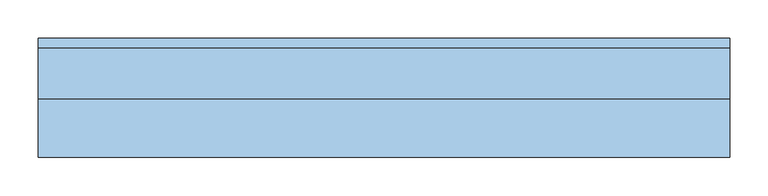
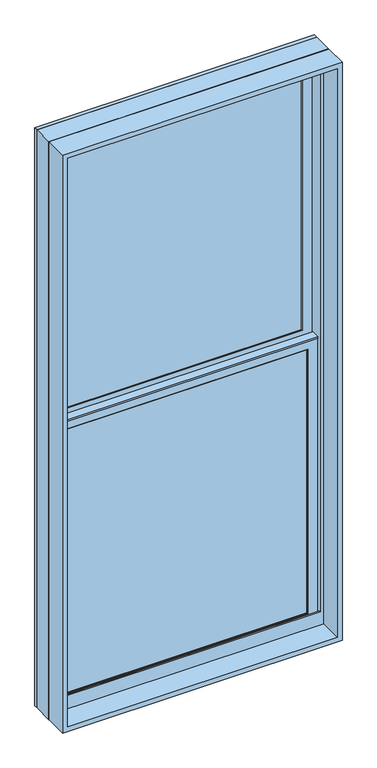
"""IFC4 building model written with IfcOpenShell, lengths in millimetres: window geometry, Window-Double_Hung-Marvin-Essential : ESDH3066."""

import ifcopenshell
import ifcopenshell.guid

model = None  # the IFC model being written
_history = None  # IfcOwnerHistory: only IFC2X3 demands one
_inside = {}  # id of a spatial element -> (the spatial element, [elements in it])
_under = {}  # id of a project, library or spatial element -> (it, [spatial elements below it])
_declared = {}  # id of a project -> (the project, [libraries it declares])
_typed = {}  # id of a type object -> (the type object, [elements of that type])
_made_of = {}  # id of a material, layer set ... -> (it, [elements and type objects made of it])


def new_model(schema):
    """Start an empty IFC model of exactly this schema.

    Asked for "IFC4X3", IfcOpenShell would pick the latest addendum, in which some entities
    have other attributes; the version numbers below select the first issue.
    IFC2X3 requires an IfcOwnerHistory on every rooted entity: one is made here for all.
    """
    global model, _history
    if schema == "IFC4X3":
        model = ifcopenshell.file(schema_version=(4, 3, 0, 0))
    else:
        model = ifcopenshell.file(schema=schema)
    _inside.clear()
    _under.clear()
    _declared.clear()
    _typed.clear()
    _made_of.clear()
    _history = None
    if model.schema == "IFC2X3":
        org = make("IfcOrganization", Name="unknown")
        user = make(
            "IfcPersonAndOrganization",
            ThePerson=make("IfcPerson", FamilyName="unknown"),
            TheOrganization=org,
        )
        app = make(
            "IfcApplication",
            ApplicationDeveloper=org,
            Version="unknown",
            ApplicationFullName="unknown",
            ApplicationIdentifier="unknown",
        )
        _history = make(
            "IfcOwnerHistory",
            OwningUser=user,
            OwningApplication=app,
            ChangeAction="ADDED",
            CreationDate=0,
        )
    return model


def make(cls, **values):
    """One entity of the class cls with the attributes given. An attribute that is None is left unset."""
    return model.create_entity(
        cls, **{name: value for name, value in values.items() if value is not None}
    )


def rooted(cls, **values):
    """An entity with a GlobalId (a new one), such as an element, a storey or a relation."""
    return make(cls, GlobalId=ifcopenshell.guid.new(), OwnerHistory=_history, **values)


def si_unit(unit_type, name, prefix=None):
    """IfcSIUnit, for example si_unit("LENGTHUNIT", "METRE", prefix="MILLI")."""
    return make("IfcSIUnit", UnitType=unit_type, Prefix=prefix, Name=name)


def assignment(units):
    """IfcUnitAssignment: the units of a project."""
    return None if units is None else make("IfcUnitAssignment", Units=units)


def point(xyz):
    """IfcCartesianPoint."""
    return None if xyz is None else make("IfcCartesianPoint", Coordinates=xyz)


def direction(xyz):
    """IfcDirection."""
    return None if xyz is None else make("IfcDirection", DirectionRatios=xyz)


def frame(location, z_axis=None, x_axis=None):
    """IfcAxis2Placement3D, a coordinate frame: its origin and axes. An axis left out is left unset."""
    return make(
        "IfcAxis2Placement3D",
        Location=point(location),
        Axis=direction(z_axis),
        RefDirection=direction(x_axis),
    )


def origin():
    """The frame at (0, 0, 0) with its axes left unset."""
    return frame((0.0, 0.0, 0.0))


def place(relative_to, where):
    """IfcLocalPlacement: puts the frame where relative to a parent placement (None: the world)."""
    return make(
        "IfcLocalPlacement", PlacementRelTo=relative_to, RelativePlacement=where
    )


def context(
    kind, dimensions, precision=None, world=None, true_north=None, identifier=None
):
    """IfcGeometricRepresentationContext, for example the 3D "Model" context."""
    return make(
        "IfcGeometricRepresentationContext",
        ContextIdentifier=identifier,
        ContextType=kind,
        CoordinateSpaceDimension=dimensions,
        Precision=precision,
        WorldCoordinateSystem=world,
        TrueNorth=true_north,
    )


def project(units=None, contexts=None):
    """IfcProject with its units and contexts."""
    return rooted(
        "IfcProject",
        Name="project",
        RepresentationContexts=contexts,
        UnitsInContext=assignment(units),
    )


def spatial(cls, under=None, at=None, **own):
    """A site, building, storey or space (cls), placed at a placement, below another one or the project."""
    s = rooted(cls, ObjectPlacement=at, **own)
    if under is not None:
        _under.setdefault(under.id(), (under, []))[1].append(s)
    return s


def polyline(points):
    """IfcPolyline through the points."""
    return make("IfcPolyline", Points=[point(p) for p in points])


def outline(outer, holes=None, kind="AREA"):
    """IfcArbitraryClosedProfileDef: a profile drawn as a closed curve; with holes, ...WithVoids."""
    if holes is None:
        return make("IfcArbitraryClosedProfileDef", ProfileType=kind, OuterCurve=outer)
    return make(
        "IfcArbitraryProfileDefWithVoids",
        ProfileType=kind,
        OuterCurve=outer,
        InnerCurves=holes,
    )


def extrude(swept, where, along, depth):
    """IfcExtrudedAreaSolid: the profile swept, set in the frame where, extruded along a direction by depth."""
    return make(
        "IfcExtrudedAreaSolid",
        SweptArea=swept,
        Position=where,
        ExtrudedDirection=direction(along),
        Depth=depth,
    )


def faces_of(points, faces, orient=None, outer=None):
    """IfcFace entities. A face is a list of loops; a loop is a list of indices into points, from 0.

    orient and outer hold one flag for each loop. By default every Orientation is true, the
    first loop of a face is its IfcFaceOuterBound and the others are IfcFaceBound.
    """
    made = []
    for i, loops in enumerate(faces):
        bounds = []
        for j, loop in enumerate(loops):
            is_outer = j == 0 if outer is None else outer[i][j]
            bounds.append(
                make(
                    "IfcFaceOuterBound" if is_outer else "IfcFaceBound",
                    Bound=make("IfcPolyLoop", Polygon=[points[k] for k in loop]),
                    Orientation=True if orient is None else orient[i][j],
                )
            )
        made.append(make("IfcFace", Bounds=bounds))
    return made


def faceted_brep(points, faces, orient=None, outer=None, voids=None):
    """IfcFacetedBrep: a solid bounded by flat faces; with voids (closed shells), ...WithVoids."""
    shared = [point(p) for p in points]
    hull = make("IfcClosedShell", CfsFaces=faces_of(shared, faces, orient, outer))
    if voids is None:
        return make("IfcFacetedBrep", Outer=hull)
    return make(
        "IfcFacetedBrepWithVoids",
        Outer=hull,
        Voids=[
            make(cls, CfsFaces=faces_of(shared, fs, o, b)) for cls, fs, o, b in voids
        ],
    )


def shape(context_of_items, identifier, shape_type, items):
    """IfcShapeRepresentation: the items that make up one representation, for example the "Body"."""
    return make(
        "IfcShapeRepresentation",
        ContextOfItems=context_of_items,
        RepresentationIdentifier=identifier,
        RepresentationType=shape_type,
        Items=items,
    )


def source(mapping_origin, context_of_items, identifier, shape_type, items):
    """IfcRepresentationMap: a shape defined once, which mapped items show again and again."""
    return make(
        "IfcRepresentationMap",
        MappingOrigin=mapping_origin,
        MappedRepresentation=shape(context_of_items, identifier, shape_type, items),
    )


def transform(
    local_origin,
    x_axis=None,
    y_axis=None,
    z_axis=None,
    scale=None,
    scale2=None,
    scale3=None,
    uniform=True,
):
    """IfcCartesianTransformationOperator3D, or its non-uniform kind. x_axis, y_axis, z_axis: its Axis1, 2, 3."""
    if uniform:
        return make(
            "IfcCartesianTransformationOperator3D",
            Axis1=direction(x_axis),
            Axis2=direction(y_axis),
            LocalOrigin=point(local_origin),
            Scale=scale,
            Axis3=direction(z_axis),
        )
    return make(
        "IfcCartesianTransformationOperator3DnonUniform",
        Axis1=direction(x_axis),
        Axis2=direction(y_axis),
        LocalOrigin=point(local_origin),
        Scale=scale,
        Axis3=direction(z_axis),
        Scale2=scale2,
        Scale3=scale3,
    )


def mapped(mapping_source, mapping_target):
    """IfcMappedItem: shows the shape of a source again, moved by a transform."""
    return make(
        "IfcMappedItem", MappingSource=mapping_source, MappingTarget=mapping_target
    )


def made_of(thing, what):
    """Note that an element or type object is made of a material, layer set ...; save() writes the relation."""
    if what is not None:
        _made_of.setdefault(what.id(), (what, []))[1].append(thing)
    return thing


def element(
    cls,
    number,
    at=None,
    inside=None,
    cuts=None,
    type_object=None,
    material=None,
    context=None,
    identifier="Body",
    shape_type=None,
    held_by="IfcProductDefinitionShape",
    body=None,
    shapes=None,
    **own,
):
    """One element of the class cls, such as IfcWall. Its Tag is "e" and its number.

    at: its placement. inside: the storey or other place that contains it. cuts: it is an
    opening in that element (IfcRelVoidsElement). A single representation is given by context,
    identifier, shape_type and body (its items); several are given by shapes. held_by: the class
    of the entity that holds the representations. save() writes the other relations.
    """
    e = rooted(cls, Tag="e%d" % number, ObjectPlacement=at, **own)
    if body is not None:
        shapes = [shape(context, identifier, shape_type, body)]
    if shapes is not None:
        e.Representation = make(held_by, Representations=shapes)
    if inside is not None:
        _inside.setdefault(inside.id(), (inside, []))[1].append(e)
    if cuts is not None:
        rooted(
            "IfcRelVoidsElement", RelatingBuildingElement=cuts, RelatedOpeningElement=e
        )
    if type_object is not None:
        _typed.setdefault(type_object.id(), (type_object, []))[1].append(e)
    return made_of(e, material)


def aggregate(whole, parts):
    """IfcRelAggregates: a whole, such as a stair, and the parts it consists of."""
    return rooted("IfcRelAggregates", RelatingObject=whole, RelatedObjects=parts)


def save(model, path):
    """Write the relations noted so far, then the file.

    IfcRelAggregates (storeys below a building ...), IfcRelContainedInSpatialStructure (elements
    in a storey), IfcRelDefinesByType, IfcRelAssociatesMaterial and IfcRelDeclares: one each for
    every whole, place, type object, material and project.
    """
    for whole, parts in _under.values():
        aggregate(whole, parts)
    for where, things in _inside.values():
        rooted(
            "IfcRelContainedInSpatialStructure",
            RelatedElements=things,
            RelatingStructure=where,
        )
    for kind, things in _typed.values():
        rooted("IfcRelDefinesByType", RelatedObjects=things, RelatingType=kind)
    for what, things in _made_of.values():
        rooted("IfcRelAssociatesMaterial", RelatedObjects=things, RelatingMaterial=what)
    for by, libraries in _declared.values():
        rooted("IfcRelDeclares", RelatingContext=by, RelatedDefinitions=libraries)
    model.write(path)


def window_3b7d5063(model_context):
    return source(origin(), model_context, "Body", "SolidModel", [
        extrude(outline(polyline([(140.7583333, 20.6375), (140.7583333, 15.875), (121.7083333, 15.875), (121.7083333, 20.6375), (140.7583333, 20.6375)])), frame((0.0, 0.0, 527.05), z_axis=(0.0, 0.0, 1.0), x_axis=(1.0, 0.0, 0.0)), (0.0, 0.0, 1.0), 908.05),
        extrude(outline(polyline([(-121.7083333, 20.6375), (-121.7083333, 15.875), (-140.7583333, 15.875), (-140.7583333, 20.6375), (-121.7083333, 20.6375)])), frame((0.0, 0.0, 527.05), z_axis=(0.0, 0.0, 1.0), x_axis=(1.0, 0.0, 0.0)), (0.0, 0.0, 1.0), 908.05),
        extrude(outline(polyline([(393.7, 20.6375), (393.7, 15.875), (-393.7, 15.875), (-393.7, 20.6375), (393.7, 20.6375)])), frame((0.0, 0.0, 971.55), z_axis=(0.0, 0.0, 1.0), x_axis=(1.0, 0.0, 0.0)), (0.0, 0.0, 1.0), 19.05),
        extrude(outline(polyline([(-140.7583333, 46.83125), (-140.7583333, 51.59375), (-121.7083333, 51.59375), (-121.7083333, 46.83125), (-140.7583333, 46.83125)])), frame((0.0, 0.0, 1473.2), z_axis=(0.0, 0.0, 1.0), x_axis=(1.0, 0.0, 0.0)), (0.0, 0.0, 1.0), 908.05),
        extrude(outline(polyline([(121.7083333, 46.83125), (121.7083333, 51.59375), (140.7583333, 51.59375), (140.7583333, 46.83125), (121.7083333, 46.83125)])), frame((0.0, 0.0, 1473.2), z_axis=(0.0, 0.0, 1.0), x_axis=(1.0, 0.0, 0.0)), (0.0, 0.0, 1.0), 908.05),
        extrude(outline(polyline([(-393.7, 46.83125), (-393.7, 51.59375), (393.7, 51.59375), (393.7, 46.83125), (-393.7, 46.83125)])), frame((0.0, 0.0, 1917.7), z_axis=(0.0, 0.0, 1.0), x_axis=(1.0, 0.0, 0.0)), (0.0, 0.0, 1.0), 19.05),
        extrude(outline(polyline([(140.7583333, 20.6375), (121.7083333, 20.6375), (121.7083333, 25.4), (140.7583333, 25.4), (140.7583333, 20.6375)])), frame((0.0, 0.0, 527.05), z_axis=(0.0, 0.0, 1.0), x_axis=(1.0, 0.0, 0.0)), (0.0, 0.0, 1.0), 908.05),
        extrude(outline(polyline([(-121.7083333, 20.6375), (-140.7583333, 20.6375), (-140.7583333, 25.4), (-121.7083333, 25.4), (-121.7083333, 20.6375)])), frame((0.0, 0.0, 527.05), z_axis=(0.0, 0.0, 1.0), x_axis=(1.0, 0.0, 0.0)), (0.0, 0.0, 1.0), 908.05),
        extrude(outline(polyline([(393.7, 20.6375), (-393.7, 20.6375), (-393.7, 25.4), (393.7, 25.4), (393.7, 20.6375)])), frame((0.0, 0.0, 971.55), z_axis=(0.0, 0.0, 1.0), x_axis=(1.0, 0.0, 0.0)), (0.0, 0.0, 1.0), 19.05),
        extrude(outline(polyline([(-140.7583333, 56.35625), (-121.7083333, 56.35625), (-121.7083333, 51.59375), (-140.7583333, 51.59375), (-140.7583333, 56.35625)])), frame((0.0, 0.0, 1473.2), z_axis=(0.0, 0.0, 1.0), x_axis=(1.0, 0.0, 0.0)), (0.0, 0.0, 1.0), 908.05),
        extrude(outline(polyline([(121.7083333, 56.35625), (140.7583333, 56.35625), (140.7583333, 51.59375), (121.7083333, 51.59375), (121.7083333, 56.35625)])), frame((0.0, 0.0, 1473.2), z_axis=(0.0, 0.0, 1.0), x_axis=(1.0, 0.0, 0.0)), (0.0, 0.0, 1.0), 908.05),
        extrude(outline(polyline([(-393.7, 56.35625), (393.7, 56.35625), (393.7, 51.59375), (-393.7, 51.59375), (-393.7, 56.35625)])), frame((0.0, 0.0, 1917.7), z_axis=(0.0, 0.0, 1.0), x_axis=(1.0, 0.0, 0.0)), (0.0, 0.0, 1.0), 19.05),
        faceted_brep([(-420.6875, 5.6780605, 1465.1351748), (-420.6875, 5.6780605, 1460.5), (420.6875, 5.6780605, 1460.5), (420.6875, 5.6780605, 1465.1351748), (-420.6875, 34.8118605, 1465.1351748), (420.6875, 34.8118605, 1465.1351748), (420.6875, 34.8118605, 1460.5), (-420.6875, 34.8118605, 1460.5), (-420.6875, 30.1625, 1460.5), (-420.6875, 30.1625, 500.0625), (-420.6875, 8.9241104, 500.0625), (-420.6875, 8.9241104, 1460.5), (420.6875, 8.9241104, 1460.5), (420.6875, 30.1625, 1460.5), (420.6875, 8.9241104, 500.0625), (420.6875, 30.1625, 500.0625), (-404.8034752, 11.90625, 1446.2034752), (-404.8034752, 30.1625, 1446.2034752), (404.8034752, 30.1625, 1446.2034752), (404.8034752, 11.90625, 1446.2034752), (-388.14375, 10.4662439, 1429.54375), (-388.14375, 11.90625, 1429.54375), (388.14375, 11.90625, 1429.54375), (388.14375, 10.4662439, 1429.54375), (389.6858834, 8.9241104, 1431.0858834), (-389.6858834, 8.9241104, 1431.0858834), (404.8034752, 30.1625, 515.9465248), (404.8034752, 11.90625, 515.9465248), (388.14375, 11.90625, 532.60625), (388.14375, 10.4662439, 532.60625), (389.6858834, 8.9241104, 531.0641166), (-404.8034752, 30.1625, 515.9465248), (-404.8034752, 11.90625, 515.9465248), (-388.14375, 11.90625, 532.60625), (-388.14375, 10.4662439, 532.60625), (-389.6858834, 8.9241104, 531.0641166)], [[[0, 1, 2, 3]], [[4, 5, 6, 7]], [[1, 0, 4, 7, 8, 9, 10, 11]], [[2, 1, 11, 12]], [[7, 6, 13, 8]], [[3, 2, 12, 14, 15, 13, 6, 5]], [[0, 3, 5, 4]], [[16, 17, 18, 19]], [[20, 21, 22, 23]], [[20, 23, 24, 25]], [[19, 18, 26, 27]], [[23, 22, 28, 29]], [[24, 23, 29, 30]], [[27, 26, 31, 32]], [[29, 28, 33, 34]], [[30, 29, 34, 35]], [[15, 14, 10, 9]], [[15, 9, 8, 13], [18, 17, 31, 26]], [[17, 16, 32, 31]], [[16, 19, 27, 32], [22, 21, 33, 28]], [[21, 20, 34, 33]], [[20, 25, 35, 34]], [[10, 14, 12, 11], [25, 24, 30, 35]]]),
        extrude(outline(polyline([(38.5955581, 1446.2125), (33.5778968, 1446.2125), (33.5778968, 1447.8), (39.9405976, 1447.8), (39.9405976, 1446.2125), (61.515625, 1446.2125), (47.6307501, 1442.8975159), (38.5955581, 1442.8975159), (38.5955581, 1446.2125)])), frame((-420.6875, 0.0, 0.0), z_axis=(1.0, 0.0, 0.0), x_axis=(0.0, 1.0, 0.0)), (0.0, 0.0, 1.0), 841.375),
        faceted_brep([(450.85, 0.0, 469.9), (450.85, 0.0, 2438.4), (-450.85, 0.0, 2438.4), (-450.85, 0.0, 469.9), (424.65625, 0.0, 531.01875), (-424.65625, 0.0, 531.01875), (-424.65625, 0.0, 2412.20625), (424.65625, 0.0, 2412.20625), (424.65625, 3.96875, 469.9), (-424.65625, 3.96875, 469.9), (-424.65625, 3.96875, 531.01875), (424.65625, 3.96875, 531.01875), (-450.85, 65.6828125, 469.9), (-424.65625, 65.6828125, 469.9), (424.65625, 65.6828125, 469.9), (450.85, 65.6828125, 469.9), (-450.85, 65.6828125, 2438.4), (450.85, 65.6828125, 2438.4), (424.65625, 65.6828125, 2412.20625), (-424.65625, 65.6828125, 2412.20625)], [[[0, 1, 2, 3], [4, 5, 6, 7]], [[8, 9, 10, 11]], [[5, 4, 11, 10]], [[0, 3, 12, 13, 9, 8, 14, 15]], [[13, 12, 16, 17, 15, 14, 18, 19]], [[13, 19, 6, 5, 10, 9]], [[7, 6, 19, 18]], [[18, 14, 8, 11, 4, 7]], [[1, 0, 15, 17]], [[2, 1, 17, 16]], [[3, 2, 16, 12]]]),
        faceted_brep([(424.65625, 30.1625, 1454.15), (423.06875, 30.1625, 1454.15), (423.06875, 30.1625, 494.2544613), (424.65625, 30.1625, 494.2544613), (-423.06875, 30.1625, 1454.15), (-424.65625, 30.1625, 1454.15), (-424.65625, 30.1625, 494.2544613), (-423.06875, 30.1625, 494.2544613), (423.06875, 63.5, 1454.15), (424.65625, 63.5, 1454.15), (424.65625, 63.5, 487.7743077), (423.06875, 63.5, 487.7743077), (-424.65625, 63.5, 1454.15), (-423.06875, 63.5, 1454.15), (-423.06875, 63.5, 487.7743077), (-424.65625, 63.5, 487.7743077), (435.9108932, 3.96875, 499.3460105), (435.9108932, 3.96875, 469.9), (435.9108932, 65.6828125, 469.9), (435.9108932, 65.6828125, 487.350012), (-435.9108932, 3.96875, 469.9), (-435.9108932, 3.96875, 499.3460105), (-435.9108932, 65.6828125, 487.350012), (-435.9108932, 65.6828125, 469.9), (435.9108932, 78.58125, 484.8428097), (-435.9108932, 78.58125, 484.8428097), (-433.8971252, 68.2348864, 486.8539391), (-415.93135, 68.2348864, 486.8539391), (-415.93135, 65.6828125, 487.350012), (415.93135, 65.6828125, 487.350012), (415.93135, 68.2348864, 486.8539391), (433.8971252, 68.2348864, 486.8539391), (-450.85, 65.6828125, 469.9), (-450.85, 78.5948249, 469.9), (450.85, 78.5948249, 469.9), (450.85, 65.6828125, 469.9), (-450.85, 78.58125, 2438.4), (450.85, 78.58125, 2438.4), (435.9108932, 78.58125, 2423.4608932), (-435.9108932, 78.58125, 2423.4608932), (-450.85, 65.6828125, 2438.4), (-433.8971252, 68.2348864, 2421.4471252), (433.8971252, 68.2348864, 2421.4471252), (415.93135, 68.2348864, 2403.48135), (-415.93135, 68.2348864, 2403.48135), (-415.93135, 65.6828125, 2403.48135), (415.93135, 65.6828125, 2403.48135), (450.85, 65.6828125, 2438.4)], [[[0, 1, 2, 3]], [[4, 5, 6, 7]], [[8, 9, 10, 11]], [[12, 13, 14, 15]], [[1, 8, 11, 2]], [[9, 0, 3, 10]], [[1, 0, 9, 8]], [[5, 4, 13, 12]], [[5, 12, 15, 6]], [[13, 4, 7, 14]], [[16, 17, 18, 19]], [[20, 21, 22, 23]], [[24, 25, 26, 27, 28, 22, 21, 16, 19, 29, 30, 31], [3, 2, 11, 10], [7, 6, 15, 14]], [[17, 16, 21, 20]], [[17, 20, 23, 32, 33, 34, 35, 18]], [[34, 33, 36, 37], [25, 24, 38, 39]], [[33, 32, 40, 36]], [[39, 41, 26, 25]], [[41, 42, 31, 30, 43, 44, 27, 26]], [[44, 45, 28, 27]], [[40, 32, 23, 22, 28, 45, 46, 29, 19, 18, 35, 47]], [[36, 40, 47, 37]], [[39, 38, 42, 41]], [[44, 43, 46, 45]], [[34, 37, 47, 35]], [[42, 38, 24, 31]], [[46, 43, 30, 29]]]),
        extrude(outline(polyline([(400.84375, 11.90625), (-400.84375, 11.90625), (-400.84375, 15.08125), (400.84375, 15.08125), (400.84375, 11.90625)])), frame((0.0, 0.0, 519.90625), z_axis=(0.0, 0.0, 1.0), x_axis=(1.0, 0.0, 0.0)), (0.0, 0.0, 1.0), 922.3375),
        extrude(outline(polyline([(400.84375, 42.8625), (-400.84375, 42.8625), (-400.84375, 46.0375), (400.84375, 46.0375), (400.84375, 42.8625)])), frame((0.0, 0.0, 1466.05625), z_axis=(0.0, 0.0, 1.0), x_axis=(1.0, 0.0, 0.0)), (0.0, 0.0, 1.0), 922.3375),
        faceted_brep([(-388.14375, 31.194477, 1429.54375), (-389.6858834, 32.7366104, 1431.0858834), (389.6858834, 32.7366104, 1431.0858834), (388.14375, 31.194477, 1429.54375), (-388.14375, 30.1625, 1429.54375), (388.14375, 30.1625, 1429.54375), (-420.6875, 32.7366104, 1462.0875), (-420.6875, 30.1625, 1462.0875), (420.6875, 30.1625, 1462.0875), (420.6875, 32.7366104, 1462.0875), (389.6858834, 32.7366104, 531.0641166), (388.14375, 31.194477, 532.60625), (388.14375, 30.1625, 532.60625), (420.6875, 30.1625, 500.0625), (420.6875, 32.7366104, 500.0625), (-389.6858834, 32.7366104, 531.0641166), (-388.14375, 31.194477, 532.60625), (-388.14375, 30.1625, 532.60625), (-420.6875, 30.1625, 500.0625), (-420.6875, 32.7366104, 500.0625)], [[[0, 1, 2, 3]], [[4, 0, 3, 5]], [[6, 7, 8, 9]], [[3, 2, 10, 11]], [[5, 3, 11, 12]], [[9, 8, 13, 14]], [[11, 10, 15, 16]], [[12, 11, 16, 17]], [[14, 13, 18, 19]], [[9, 14, 19, 6], [1, 15, 10, 2]], [[16, 15, 1, 0]], [[17, 16, 0, 4]], [[7, 18, 13, 8], [5, 12, 17, 4]], [[19, 18, 7, 6]]]),
        faceted_brep([(-404.8034752, 42.8625, 2392.3534752), (-404.8034752, 61.11875, 2392.3534752), (404.8034752, 61.11875, 2392.3534752), (404.8034752, 42.8625, 2392.3534752), (-388.14375, 41.4224939, 2375.69375), (-388.14375, 42.8625, 2375.69375), (388.14375, 42.8625, 2375.69375), (388.14375, 41.4224939, 2375.69375), (-389.6858834, 39.8803604, 2377.2358834), (389.6858834, 39.8803604, 2377.2358834), (-420.6875, 61.11875, 2408.2375), (-420.6875, 39.8803604, 2408.2375), (420.6875, 39.8803604, 2408.2375), (420.6875, 61.11875, 2408.2375), (404.8034752, 61.11875, 1462.0965248), (404.8034752, 42.8625, 1462.0965248), (388.14375, 42.8625, 1478.75625), (388.14375, 41.4224939, 1478.75625), (389.6858834, 39.8803604, 1477.2141166), (420.6875, 39.8803604, 1446.2125), (420.6875, 61.11875, 1446.2125), (-404.8034752, 61.11875, 1462.0965248), (-404.8034752, 42.8625, 1462.0965248), (-388.14375, 42.8625, 1478.75625), (-388.14375, 41.4224939, 1478.75625), (-389.6858834, 39.8803604, 1477.2141166), (-420.6875, 39.8803604, 1446.2125), (-420.6875, 61.11875, 1446.2125)], [[[0, 1, 2, 3]], [[4, 5, 6, 7]], [[8, 4, 7, 9]], [[10, 11, 12, 13]], [[3, 2, 14, 15]], [[7, 6, 16, 17]], [[9, 7, 17, 18]], [[13, 12, 19, 20]], [[15, 14, 21, 22]], [[17, 16, 23, 24]], [[18, 17, 24, 25]], [[20, 19, 26, 27]], [[13, 20, 27, 10], [1, 21, 14, 2]], [[22, 21, 1, 0]], [[3, 15, 22, 0], [5, 23, 16, 6]], [[24, 23, 5, 4]], [[25, 24, 4, 8]], [[11, 26, 19, 12], [9, 18, 25, 8]], [[27, 26, 11, 10]]]),
        faceted_brep([(-420.6875, 61.11875, 1446.2125), (-420.6875, 63.6928604, 1446.2125), (420.6875, 63.6928604, 1446.2125), (420.6875, 61.11875, 1446.2125), (-388.14375, 62.150727, 1478.75625), (-388.14375, 61.11875, 1478.75625), (388.14375, 61.11875, 1478.75625), (388.14375, 62.150727, 1478.75625), (-389.6858834, 63.6928604, 1477.2141166), (389.6858834, 63.6928604, 1477.2141166), (420.6875, 63.6928604, 2408.2375), (420.6875, 61.11875, 2408.2375), (388.14375, 61.11875, 2375.69375), (388.14375, 62.150727, 2375.69375), (389.6858834, 63.6928604, 2377.2358834), (-420.6875, 63.6928604, 2408.2375), (-420.6875, 61.11875, 2408.2375), (-388.14375, 61.11875, 2375.69375), (-388.14375, 62.150727, 2375.69375), (-389.6858834, 63.6928604, 2377.2358834)], [[[0, 1, 2, 3]], [[4, 5, 6, 7]], [[8, 4, 7, 9]], [[3, 2, 10, 11]], [[7, 6, 12, 13]], [[9, 7, 13, 14]], [[11, 10, 15, 16]], [[13, 12, 17, 18]], [[14, 13, 18, 19]], [[16, 15, 1, 0]], [[3, 11, 16, 0], [5, 17, 12, 6]], [[18, 17, 5, 4]], [[19, 18, 4, 8]], [[1, 15, 10, 2], [9, 14, 19, 8]]]),
        extrude(outline(polyline([(400.84375, 26.19375), (-400.84375, 26.19375), (-400.84375, 30.1625), (400.84375, 30.1625), (400.84375, 26.19375)])), frame((0.0, 0.0, 519.90625), z_axis=(0.0, 0.0, 1.0), x_axis=(1.0, 0.0, 0.0)), (0.0, 0.0, 1.0), 922.3375),
        extrude(outline(polyline([(400.84375, 57.15), (-400.84375, 57.15), (-400.84375, 61.11875), (400.84375, 61.11875), (400.84375, 57.15)])), frame((0.0, 0.0, 1466.05625), z_axis=(0.0, 0.0, 1.0), x_axis=(1.0, 0.0, 0.0)), (0.0, 0.0, 1.0), 922.3375),
        extrude(outline(polyline([(2438.4, 450.85), (2438.4, -450.85), (469.9, -450.85), (469.9, 450.85), (2438.4, 450.85)]), holes=[polyline([(2422.525, 434.975), (485.775, 434.975), (485.775, -434.975), (2422.525, -434.975), (2422.525, 434.975)])]), frame((0.0, -76.2, 0.0), z_axis=(0.0, 1.0, 0.0), x_axis=(0.0, 0.0, 1.0)), (0.0, 0.0, 1.0), 75.40625),
    ])


if __name__ == "__main__":
    model = new_model("IFC4")
    model_context = context("Model", 3, world=origin())
    ifc_project = project(units=[si_unit("LENGTHUNIT", "METRE", prefix="MILLI")], contexts=[model_context])
    site = spatial("IfcSite", under=ifc_project)
    building = spatial("IfcBuilding", under=site)
    placement = place(None, origin())
    window_shape = window_3b7d5063(model_context)
    element("IfcWindow", 1, ObjectType="Window-Double_Hung-Marvin-Essential : ESDH3066", at=placement, inside=building, context=model_context, shape_type="MappedRepresentation", body=[
        mapped(window_shape, transform((0.0, 0.0, 0.0), x_axis=(1.0, 0.0, 0.0), y_axis=(0.0, 1.0, 0.0), z_axis=(0.0, 0.0, 1.0))),
    ])
    save(model, "model.ifc")

# Revit data of these elements
# Type "Window-Double_Hung-Marvin-Essential : ESDH3066"
#   Type Mark = "86"
#   Window Type = "Essential Double Hung"
#   Product data url = "https://bimobject.com/marvin-windows-and-doors/product/marvin-dhwau"
#   Product Guid = "c4a96547-874c-4385-91dc-a058adc19d98"
#   Frame = "All Ultrex"
#   Egress Window = "Yes"
#   URL = "www.marvin.com"
#   Model = "ESDH3066"
#   Manufacturer = "Marvin Windows and Doors"
#   Label Egress = "EGRESS WDW"
#   Glass Type = "IG Low E II with Argon"
#   Design Pressure = "DP40"
#   Description = "3678 DBHG"
#   Analytic Construction = "<None>"
#   Prairie Corner Width = 0' - 4"
#   Prairie Corner Height = 0' - 4"
#   Egress Width = 2' - 8 9/16"
#   Egress Height = 2' - 10 27/128"
#   Rough Width = 3' - 0"
#   Rough Height = 6' - 6"
#   Nominal Width = 3' - 0"
#   Nominal Height = 6' - 6"
#   Inset to Installation Flange [instance default] = 0' - 1"
#   Height = 6' - 5 1/2"
#   Egress Area = 7.73607 SF
#   Default Head Height = 8' - 0"
#   Width = 2' - 11 1/2"
#   Daylight Area = 14.9894 SF
#   DLO Width = 2' - 6 9/16"
#   DLO Height = 2' - 11 5/16"
#   Muntins Top Sash = yes
#   Lites Wide Top Sash = 3
#   Lites Wide Bottom Sash = 3
#   Lites High Top Sash = 2
#   Lites High Bottom Sash = 2
#   Lite Cut Prairie 9 = no
#   Lite Cut HV Grid = yes
#   Muntins Bottom Sash = yes
#   Label Visibility = no
#   Jamb Extension Visibility = yes
#   Edition number = 1
#   Interior Material = Ultrex-Marvin-Stonewhite
#   Glazing Material = Glass-Marvin-IG Low E II with Argon
#   Cladding Material = Ultrex-Marvin-Pebblegray
#   Wall Closure = (empty or 0)
#   Assembly Code = ""
# Element 1 (IfcWindow, "Window-Double_Hung-Marvin-Essential : ESDH3066")
#   Materials on its faces: "Ultrex-Marvin-Pebblegray", "Ultrex-Marvin-Stonewhite", "Glass-Marvin-IG Low E II with Argon"
# Materials
#   "Ultrex-Marvin-Stonewhite": class "Paint", colour RGB 250 251 245, transparency 0
#   "Glass-Marvin-IG Low E II with Argon": class "Glass", colour RGB 0 128 192, transparency 0.85
#   "Ultrex-Marvin-Pebblegray": class "Paint", colour RGB 189 185 173, transparency 0
